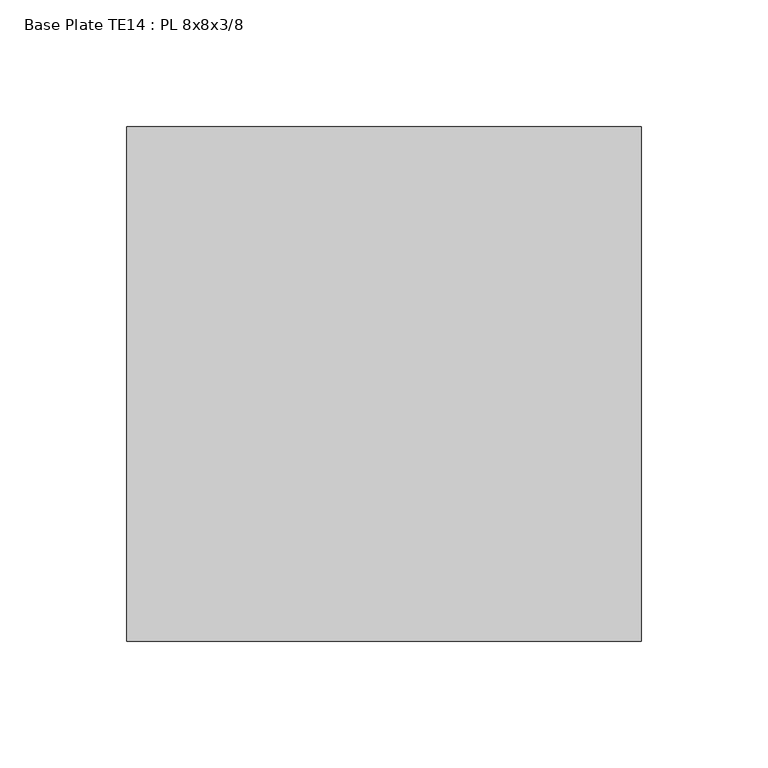
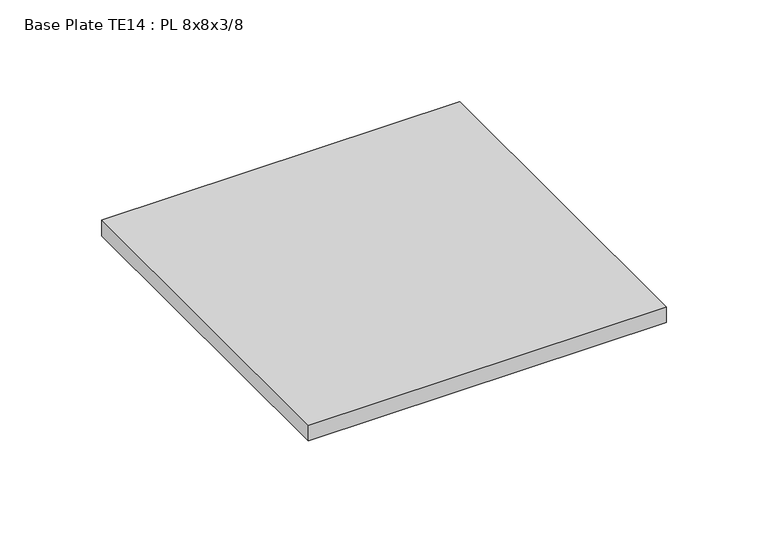
"""IFC4 building model written with IfcOpenShell, lengths in millimetres: proxy geometry, Base Plate TE14 : PL 8x8x3/8."""

from ifc_helpers import new_model, si_unit, frame, origin, place, context, project, spatial, polyline, outline, extrude, source, transform, mapped, element, save


def base_plate_te14_pl_8x8x3_8_4141263b(model_context):
    return source(origin(), model_context, "Body", "SweptSolid", [
        extrude(outline(polyline([(587365.8770246, -536468.3913841), (587365.8770246, -536265.1913841), (587569.0770246, -536265.1913841), (587569.0770246, -536468.3913841), (587365.8770246, -536468.3913841)])), frame((0.0, 0.0, 19.05), z_axis=(0.0, 0.0, 1.0), x_axis=(1.0, 0.0, 0.0)), (0.0, 0.0, 1.0), 9.525),
    ])


if __name__ == "__main__":
    model = new_model("IFC4")
    model_context = context("Model", 3, world=origin())
    ifc_project = project(units=[si_unit("LENGTHUNIT", "METRE", prefix="MILLI")], contexts=[model_context])
    site = spatial("IfcSite", under=ifc_project)
    building = spatial("IfcBuilding", under=site)
    placement = place(None, origin())
    base_plate_te14_pl_8x8x3_8_shape = base_plate_te14_pl_8x8x3_8_4141263b(model_context)
    element("IfcBuildingElementProxy", 1, Name="Base Plate TE14 : PL 8x8x3/8", ObjectType="Base Plate TE14 : PL 8x8x3/8", at=placement, inside=building, context=model_context, shape_type="MappedRepresentation", body=[
        mapped(base_plate_te14_pl_8x8x3_8_shape, transform((0.0, 0.0, 0.0), x_axis=(1.0, 0.0, 0.0), y_axis=(0.0, 1.0, 0.0), z_axis=(0.0, 0.0, 1.0))),
    ])
    save(model, "model.ifc")

# Revit data of these elements
# Element 1 (IfcBuildingElementProxy, "Base Plate TE14 : PL 8x8x3/8")
#   Materials on its faces: "GALV. STL BASE PLATE"
# Materials
#   "GALV. STL BASE PLATE": class "Generic", colour RGB 211 211 207, transparency 0, Cost = 0
